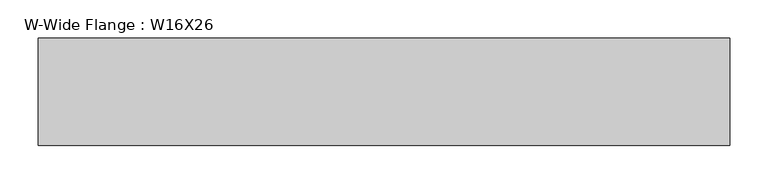
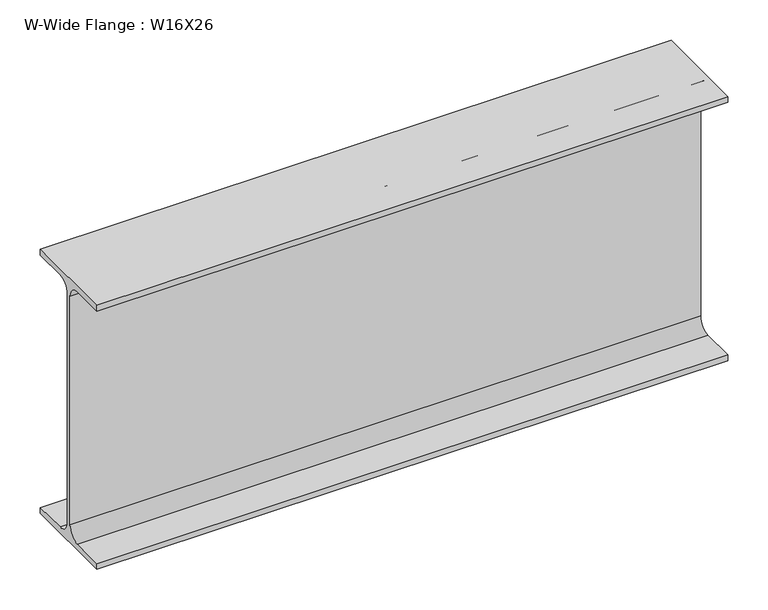
"""IFC4 building model written with IfcOpenShell, lengths in millimetres: beam geometry, W-Wide Flange : W16X26."""

from ifc_helpers import new_model, si_unit, point, frame, frame_2d, origin, place, context, project, spatial, polyline, circle_curve, trimmed, segment, composite_curve, outline, extrude, source, transform, mapped, element, save


def w_wide_flange_w16x26_3b22cc20(model_context):
    return source(origin(), model_context, "Body", "SweptSolid", [
        extrude(outline(composite_curve([segment(polyline([(69.85, -190.5496094), (69.85, -199.2808594), (-69.85, -199.2808594), (-69.85, -190.5496094), (-21.43125, -190.5496094)]), True, "CONTINUOUS"), segment(trimmed(circle_curve(frame_2d((-21.43125, -172.2933594)), 18.25625), [point((-21.43125, -190.5496094))], [point((-3.175, -172.2933594))], True, "CARTESIAN"), True, "CONTINUOUS"), segment(polyline([(-3.175, -172.2933594), (-3.175, 172.2933594)]), True, "CONTINUOUS"), segment(trimmed(circle_curve(frame_2d((-21.43125, 172.2933594)), 18.25625), [point((-3.175, 172.2933594))], [point((-21.43125, 190.5496094))], True, "CARTESIAN"), True, "CONTINUOUS"), segment(polyline([(-21.43125, 190.5496094), (-69.85, 190.5496094), (-69.85, 199.2808594), (69.85, 199.2808594), (69.85, 190.5496094), (21.43125, 190.5496094)]), True, "CONTINUOUS"), segment(trimmed(circle_curve(frame_2d((21.43125, 172.2933594)), 18.25625), [point((21.43125, 190.5496094))], [point((3.175, 172.2933594))], True, "CARTESIAN"), True, "CONTINUOUS"), segment(polyline([(3.175, 172.2933594), (3.175, -172.2933594)]), True, "CONTINUOUS"), segment(trimmed(circle_curve(frame_2d((21.43125, -172.2933594)), 18.25625), [point((3.175, -172.2933594))], [point((21.43125, -190.5496094))], True, "CARTESIAN"), True, "CONTINUOUS"), segment(polyline([(21.43125, -190.5496094), (69.85, -190.5496094)]), True, "CONTINUOUS")], self_intersect=False)), frame((-469.9, 0.0, 0.0), z_axis=(1.0, 0.0, 0.0), x_axis=(0.0, 1.0, 0.0)), (0.0, 0.0, 1.0), 900.43),
    ])


if __name__ == "__main__":
    model = new_model("IFC4")
    model_context = context("Model", 3, world=origin())
    ifc_project = project(units=[si_unit("LENGTHUNIT", "METRE", prefix="MILLI")], contexts=[model_context])
    site = spatial("IfcSite", under=ifc_project)
    building = spatial("IfcBuilding", under=site)
    placement = place(None, origin())
    w_wide_flange_w16x26_shape = w_wide_flange_w16x26_3b22cc20(model_context)
    element("IfcBeam", 1, ObjectType="W-Wide Flange : W16X26", at=placement, inside=building, context=model_context, shape_type="MappedRepresentation", body=[
        mapped(w_wide_flange_w16x26_shape, transform((0.0, 0.0, 0.0), x_axis=(1.0, 0.0, 0.0), y_axis=(0.0, 1.0, 0.0), z_axis=(0.0, 0.0, 1.0))),
    ])
    save(model, "model.ifc")

# Revit data of these elements
# Type "W-Wide Flange : W16X26"
#   Assembly Code = "B10"
#   W = 26
#   Start Extension Calculation [instance default] = 10' - 0"
#   Start Extension [instance default] = -0' - 0 1/2"
#   End Extension Calculation [instance default] = 10' - 0"
#   End Extension [instance default] = -0' - 0 1/2"
#   Length [instance default] = 5' - 0"
#   bf = 0' - 5 1/2"
#   d = 1' - 3 177/256"
#   k = 0' - 1 1/16"
#   k2 = 0' - 0 23/32"
#   tf = 0' - 0 11/32"
#   tw = 0' - 0 1/4"
#   A = 0.05 SF
#   Beam Material [instance default] = Metal - Steel - ASTM A992
# Element 1 (IfcBeam, "W-Wide Flange : W16X26")
#   Materials on its faces: "Metal - Steel - ASTM A992"
# Materials
#   "Metal - Steel - ASTM A992": class "Metal", colour RGB 128 0 0, transparency 0
